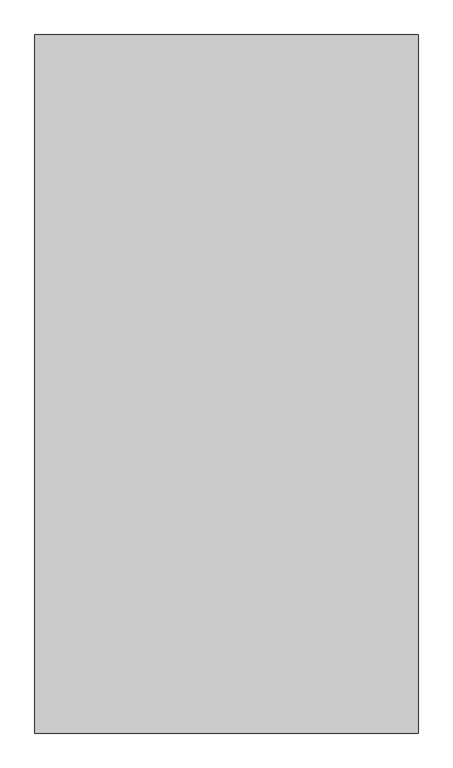
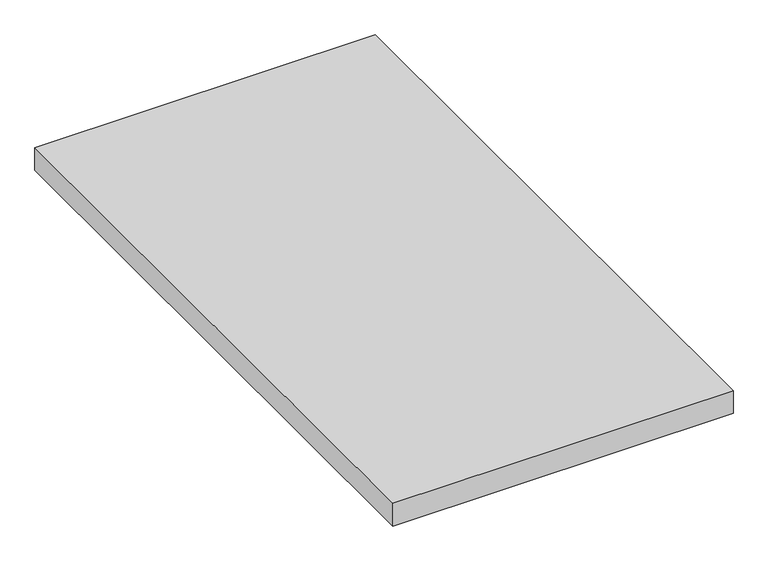
"""IFC4 building model written with IfcOpenShell, lengths in millimetres: proxy geometry, Deckendurchbruch."""

from ifc_helpers import new_model, si_unit, origin, origin_with_axes, place, context, project, spatial, polyline, outline, extrude, source, transform, mapped, element, save


def generic_models_fb710a73(model_context):
    return source(origin(), model_context, "Body", "SweptSolid", [
        extrude(outline(polyline([(3800.0, 0.0), (0.0, 0.0), (0.0, 6925.0), (3800.0, 6925.0), (3800.0, 0.0)])), origin_with_axes(), (0.0, 0.0, 1.0), 270.0),
    ])


if __name__ == "__main__":
    model = new_model("IFC4")
    model_context = context("Model", 3, world=origin())
    ifc_project = project(units=[si_unit("LENGTHUNIT", "METRE", prefix="MILLI")], contexts=[model_context])
    site = spatial("IfcSite", under=ifc_project)
    building = spatial("IfcBuilding", under=site)
    placement = place(None, origin())
    generic_models_shape = generic_models_fb710a73(model_context)
    element("IfcBuildingElementProxy", 1, Name="Deckendurchbruch", ObjectType="Deckendurchbruch", at=placement, inside=building, context=model_context, shape_type="MappedRepresentation", body=[
        mapped(generic_models_shape, transform((0.0, 0.0, 0.0), x_axis=(1.0, 0.0, 0.0), y_axis=(0.0, 1.0, 0.0), z_axis=(0.0, 0.0, 1.0))),
    ])
    save(model, "model.ifc")

# Revit data of these elements
# Element 1 (IfcBuildingElementProxy, "Deckendurchbruch")
#   Materials on its faces: "IfcOpeningElement"
# Materials
#   "IfcOpeningElement": class "Unassigned", colour RGB 255 165 0, transparency 0.75
